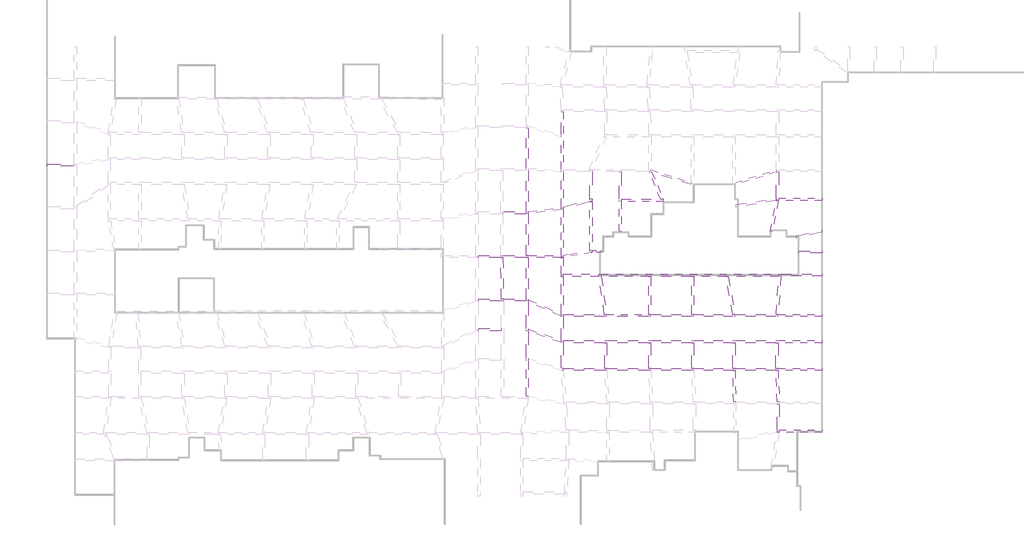
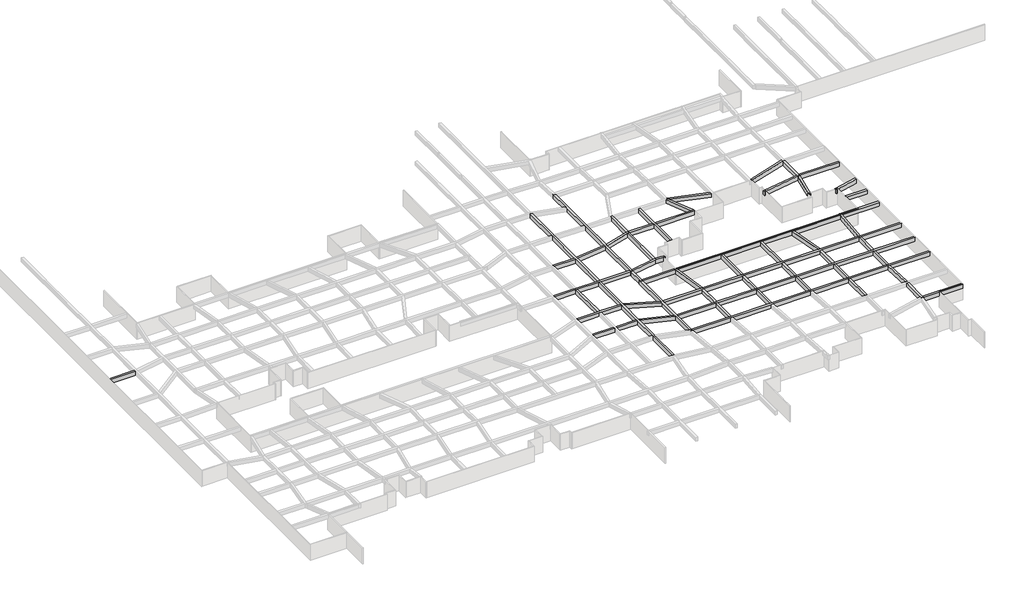
# One storey, part 13 of 45: 50 beams.
"""IFC4 building model written with IfcOpenShell, lengths in millimetres."""

import ifcopenshell
import ifcopenshell.guid

model = None  # the IFC model being written
_history = None  # IfcOwnerHistory: only IFC2X3 demands one
_inside = {}  # id of a spatial element -> (the spatial element, [elements in it])
_under = {}  # id of a project, library or spatial element -> (it, [spatial elements below it])
_declared = {}  # id of a project -> (the project, [libraries it declares])
_typed = {}  # id of a type object -> (the type object, [elements of that type])
_made_of = {}  # id of a material, layer set ... -> (it, [elements and type objects made of it])


def new_model(schema):
    """Start an empty IFC model of exactly this schema.

    Asked for "IFC4X3", IfcOpenShell would pick the latest addendum, in which some entities
    have other attributes; the version numbers below select the first issue.
    IFC2X3 requires an IfcOwnerHistory on every rooted entity: one is made here for all.
    """
    global model, _history
    if schema == "IFC4X3":
        model = ifcopenshell.file(schema_version=(4, 3, 0, 0))
    else:
        model = ifcopenshell.file(schema=schema)
    _inside.clear()
    _under.clear()
    _declared.clear()
    _typed.clear()
    _made_of.clear()
    _history = None
    if model.schema == "IFC2X3":
        org = make("IfcOrganization", Name="unknown")
        user = make(
            "IfcPersonAndOrganization",
            ThePerson=make("IfcPerson", FamilyName="unknown"),
            TheOrganization=org,
        )
        app = make(
            "IfcApplication",
            ApplicationDeveloper=org,
            Version="unknown",
            ApplicationFullName="unknown",
            ApplicationIdentifier="unknown",
        )
        _history = make(
            "IfcOwnerHistory",
            OwningUser=user,
            OwningApplication=app,
            ChangeAction="ADDED",
            CreationDate=0,
        )
    return model


def make(cls, **values):
    """One entity of the class cls with the attributes given. An attribute that is None is left unset."""
    return model.create_entity(
        cls, **{name: value for name, value in values.items() if value is not None}
    )


def rooted(cls, **values):
    """An entity with a GlobalId (a new one), such as an element, a storey or a relation."""
    return make(cls, GlobalId=ifcopenshell.guid.new(), OwnerHistory=_history, **values)


def si_unit(unit_type, name, prefix=None):
    """IfcSIUnit, for example si_unit("LENGTHUNIT", "METRE", prefix="MILLI")."""
    return make("IfcSIUnit", UnitType=unit_type, Prefix=prefix, Name=name)


def assignment(units):
    """IfcUnitAssignment: the units of a project."""
    return None if units is None else make("IfcUnitAssignment", Units=units)


def point(xyz):
    """IfcCartesianPoint."""
    return None if xyz is None else make("IfcCartesianPoint", Coordinates=xyz)


def direction(xyz):
    """IfcDirection."""
    return None if xyz is None else make("IfcDirection", DirectionRatios=xyz)


def frame(location, z_axis=None, x_axis=None):
    """IfcAxis2Placement3D, a coordinate frame: its origin and axes. An axis left out is left unset."""
    return make(
        "IfcAxis2Placement3D",
        Location=point(location),
        Axis=direction(z_axis),
        RefDirection=direction(x_axis),
    )


def origin():
    """The frame at (0, 0, 0) with its axes left unset."""
    return frame((0.0, 0.0, 0.0))


def place(relative_to, where):
    """IfcLocalPlacement: puts the frame where relative to a parent placement (None: the world)."""
    return make(
        "IfcLocalPlacement", PlacementRelTo=relative_to, RelativePlacement=where
    )


def context(
    kind, dimensions, precision=None, world=None, true_north=None, identifier=None
):
    """IfcGeometricRepresentationContext, for example the 3D "Model" context."""
    return make(
        "IfcGeometricRepresentationContext",
        ContextIdentifier=identifier,
        ContextType=kind,
        CoordinateSpaceDimension=dimensions,
        Precision=precision,
        WorldCoordinateSystem=world,
        TrueNorth=true_north,
    )


def project(units=None, contexts=None):
    """IfcProject with its units and contexts."""
    return rooted(
        "IfcProject",
        Name="project",
        RepresentationContexts=contexts,
        UnitsInContext=assignment(units),
    )


def spatial(cls, under=None, at=None, **own):
    """A site, building, storey or space (cls), placed at a placement, below another one or the project."""
    s = rooted(cls, ObjectPlacement=at, **own)
    if under is not None:
        _under.setdefault(under.id(), (under, []))[1].append(s)
    return s


def polyline(points):
    """IfcPolyline through the points."""
    return make("IfcPolyline", Points=[point(p) for p in points])


def outline(outer, holes=None, kind="AREA"):
    """IfcArbitraryClosedProfileDef: a profile drawn as a closed curve; with holes, ...WithVoids."""
    if holes is None:
        return make("IfcArbitraryClosedProfileDef", ProfileType=kind, OuterCurve=outer)
    return make(
        "IfcArbitraryProfileDefWithVoids",
        ProfileType=kind,
        OuterCurve=outer,
        InnerCurves=holes,
    )


def extrude(swept, where, along, depth):
    """IfcExtrudedAreaSolid: the profile swept, set in the frame where, extruded along a direction by depth."""
    return make(
        "IfcExtrudedAreaSolid",
        SweptArea=swept,
        Position=where,
        ExtrudedDirection=direction(along),
        Depth=depth,
    )


def faces_of(points, faces, orient=None, outer=None):
    """IfcFace entities. A face is a list of loops; a loop is a list of indices into points, from 0.

    orient and outer hold one flag for each loop. By default every Orientation is true, the
    first loop of a face is its IfcFaceOuterBound and the others are IfcFaceBound.
    """
    made = []
    for i, loops in enumerate(faces):
        bounds = []
        for j, loop in enumerate(loops):
            is_outer = j == 0 if outer is None else outer[i][j]
            bounds.append(
                make(
                    "IfcFaceOuterBound" if is_outer else "IfcFaceBound",
                    Bound=make("IfcPolyLoop", Polygon=[points[k] for k in loop]),
                    Orientation=True if orient is None else orient[i][j],
                )
            )
        made.append(make("IfcFace", Bounds=bounds))
    return made


def faceted_brep(points, faces, orient=None, outer=None, voids=None):
    """IfcFacetedBrep: a solid bounded by flat faces; with voids (closed shells), ...WithVoids."""
    shared = [point(p) for p in points]
    hull = make("IfcClosedShell", CfsFaces=faces_of(shared, faces, orient, outer))
    if voids is None:
        return make("IfcFacetedBrep", Outer=hull)
    return make(
        "IfcFacetedBrepWithVoids",
        Outer=hull,
        Voids=[
            make(cls, CfsFaces=faces_of(shared, fs, o, b)) for cls, fs, o, b in voids
        ],
    )


def shape(context_of_items, identifier, shape_type, items):
    """IfcShapeRepresentation: the items that make up one representation, for example the "Body"."""
    return make(
        "IfcShapeRepresentation",
        ContextOfItems=context_of_items,
        RepresentationIdentifier=identifier,
        RepresentationType=shape_type,
        Items=items,
    )


def source(mapping_origin, context_of_items, identifier, shape_type, items):
    """IfcRepresentationMap: a shape defined once, which mapped items show again and again."""
    return make(
        "IfcRepresentationMap",
        MappingOrigin=mapping_origin,
        MappedRepresentation=shape(context_of_items, identifier, shape_type, items),
    )


def transform(
    local_origin,
    x_axis=None,
    y_axis=None,
    z_axis=None,
    scale=None,
    scale2=None,
    scale3=None,
    uniform=True,
):
    """IfcCartesianTransformationOperator3D, or its non-uniform kind. x_axis, y_axis, z_axis: its Axis1, 2, 3."""
    if uniform:
        return make(
            "IfcCartesianTransformationOperator3D",
            Axis1=direction(x_axis),
            Axis2=direction(y_axis),
            LocalOrigin=point(local_origin),
            Scale=scale,
            Axis3=direction(z_axis),
        )
    return make(
        "IfcCartesianTransformationOperator3DnonUniform",
        Axis1=direction(x_axis),
        Axis2=direction(y_axis),
        LocalOrigin=point(local_origin),
        Scale=scale,
        Axis3=direction(z_axis),
        Scale2=scale2,
        Scale3=scale3,
    )


def mapped(mapping_source, mapping_target):
    """IfcMappedItem: shows the shape of a source again, moved by a transform."""
    return make(
        "IfcMappedItem", MappingSource=mapping_source, MappingTarget=mapping_target
    )


def made_of(thing, what):
    """Note that an element or type object is made of a material, layer set ...; save() writes the relation."""
    if what is not None:
        _made_of.setdefault(what.id(), (what, []))[1].append(thing)
    return thing


def element(
    cls,
    number,
    at=None,
    inside=None,
    cuts=None,
    type_object=None,
    material=None,
    context=None,
    identifier="Body",
    shape_type=None,
    held_by="IfcProductDefinitionShape",
    body=None,
    shapes=None,
    **own,
):
    """One element of the class cls, such as IfcWall. Its Tag is "e" and its number.

    at: its placement. inside: the storey or other place that contains it. cuts: it is an
    opening in that element (IfcRelVoidsElement). A single representation is given by context,
    identifier, shape_type and body (its items); several are given by shapes. held_by: the class
    of the entity that holds the representations. save() writes the other relations.
    """
    e = rooted(cls, Tag="e%d" % number, ObjectPlacement=at, **own)
    if body is not None:
        shapes = [shape(context, identifier, shape_type, body)]
    if shapes is not None:
        e.Representation = make(held_by, Representations=shapes)
    if inside is not None:
        _inside.setdefault(inside.id(), (inside, []))[1].append(e)
    if cuts is not None:
        rooted(
            "IfcRelVoidsElement", RelatingBuildingElement=cuts, RelatedOpeningElement=e
        )
    if type_object is not None:
        _typed.setdefault(type_object.id(), (type_object, []))[1].append(e)
    return made_of(e, material)


def aggregate(whole, parts):
    """IfcRelAggregates: a whole, such as a stair, and the parts it consists of."""
    return rooted("IfcRelAggregates", RelatingObject=whole, RelatedObjects=parts)


def save(model, path):
    """Write the relations noted so far, then the file.

    IfcRelAggregates (storeys below a building ...), IfcRelContainedInSpatialStructure (elements
    in a storey), IfcRelDefinesByType, IfcRelAssociatesMaterial and IfcRelDeclares: one each for
    every whole, place, type object, material and project.
    """
    for whole, parts in _under.values():
        aggregate(whole, parts)
    for where, things in _inside.values():
        rooted(
            "IfcRelContainedInSpatialStructure",
            RelatedElements=things,
            RelatingStructure=where,
        )
    for kind, things in _typed.values():
        rooted("IfcRelDefinesByType", RelatedObjects=things, RelatingType=kind)
    for what, things in _made_of.values():
        rooted("IfcRelAssociatesMaterial", RelatedObjects=things, RelatingMaterial=what)
    for by, libraries in _declared.values():
        rooted("IfcRelDeclares", RelatingContext=by, RelatedDefinitions=libraries)
    model.write(path)


def kl_beam_52378874(model_context):
    return source(origin(), model_context, "Body", "SweptSolid", [
        extrude(outline(polyline([(2121.5, 200.0), (2121.5, -200.0), (-2121.5, -200.0), (-2121.5, 200.0), (2121.5, 200.0)])), frame((0.0, 0.0, -400.0), z_axis=(0.0, 0.0, 1.0), x_axis=(1.0, 0.0, 0.0)), (0.0, 0.0, 1.0), 800.0),
    ])


def kl_beam_6fd21aec(model_context):
    return source(origin(), model_context, "Body", "SweptSolid", [
        extrude(outline(polyline([(2394.5, 200.0), (2394.5, -200.0), (-2394.5, -200.0), (-2394.5, 200.0), (2394.5, 200.0)])), frame((0.0, 0.0, -400.0), z_axis=(0.0, 0.0, 1.0), x_axis=(1.0, 0.0, 0.0)), (0.0, 0.0, 1.0), 800.0),
    ])


model = new_model("IFC4")

# Units and contexts
model_context = context("Model", 3, world=origin())
ifc_project = project(units=[si_unit("LENGTHUNIT", "METRE", prefix="MILLI")], contexts=[model_context])

# Site, building, storey
site = spatial("IfcSite", under=ifc_project)
building = spatial("IfcBuilding", under=site)
storey = spatial("IfcBuildingStorey", under=building, Name="户型图", Elevation=0.0)

# Beams
placement = place(None, origin())
element("IfcBeam", 1, ObjectType="KL_beam", at=placement, inside=storey, context=model_context, shape_type="SweptSolid", body=[
    extrude(outline(polyline([(-145640.2964556, -126946.3745528), (-145640.2964556, -126546.3745528), (-140635.0712547, -126546.3745528), (-140635.0712547, -126946.3745528), (-145640.2964556, -126946.3745528)])), frame((0.0, 0.0, 2500.0), z_axis=(0.0, 0.0, 1.0), x_axis=(1.0, 0.0, 0.0)), (0.0, 0.0, 1.0), 800.0),
])
element("IfcBeam", 2, ObjectType="KL_beam", at=placement, inside=storey, context=model_context, shape_type="SweptSolid", body=[
    extrude(outline(polyline([(-62877.6696197, -135611.286122), (-62877.6696197, -135211.286122), (-58630.7823984, -135211.286122), (-58630.7823984, -135611.286122), (-62877.6696197, -135611.286122)])), frame((0.0, 0.0, 2500.0), z_axis=(0.0, 0.0, 1.0), x_axis=(1.0, 0.0, 0.0)), (0.0, 0.0, 1.0), 800.0),
])
element("IfcBeam", 3, ObjectType="KL_beam", at=placement, inside=storey, context=model_context, shape_type="SweptSolid", body=[
    extrude(outline(polyline([(-58230.7823984, -135588.2311749), (-58230.7823984, -135185.2272447), (-52297.3620817, -134456.6948365), (-52297.3620817, -134859.6987667), (-58230.7823984, -135588.2311749)])), frame((0.0, 0.0, 2500.0), z_axis=(0.0, 0.0, 1.0), x_axis=(1.0, 0.0, 0.0)), (0.0, 0.0, 1.0), 800.0),
])
element("IfcBeam", 4, ObjectType="KL_beam", at=placement, inside=storey, context=model_context, shape_type="Brep", body=[
    faceted_brep([(-46687.6738698, -132877.4716384, 3300.0), (-46687.6738698, -132877.4716384, 2500.0), (-47087.6738698, -132992.1697928, 2500.0), (-51897.3620817, -134371.3256945, 2500.0), (-51897.3620817, -134371.3256945, 3300.0), (-47087.6738698, -132992.1697928, 3300.0), (-46687.6738698, -132942.8806028, 3300.0), (-46687.6738698, -133293.5914128, 3300.0), (-46687.6738698, -133293.5914128, 2500.0), (-46687.6738698, -132942.8806028, 2500.0), (-51897.3620817, -134787.4454688, 2500.0), (-51897.3620817, -134787.4454688, 3300.0), (-47087.4987798, -133408.2393608, 3300.0), (-46859.5657029, -133342.8806028, 3300.0), (-47087.4987798, -133408.2393608, 2500.0), (-46859.5657029, -133342.8806028, 2500.0)], [[[0, 1, 2, 3, 4, 5]], [[0, 6, 7, 8, 9, 1]], [[4, 3, 10, 11]], [[7, 6, 0, 5, 4, 11, 12, 13]], [[8, 7, 13, 12, 11, 10, 14, 15]], [[1, 9, 8, 15, 14, 10, 3, 2]]]),
])
element("IfcBeam", 5, ObjectType="KL_beam", at=placement, inside=storey, context=model_context, shape_type="Brep", body=[
    faceted_brep([(-46687.6738698, -127542.8806028, 3300.0), (-46784.6415945, -127542.8806028, 3300.0), (-47087.6738698, -127542.8806028, 3300.0), (-47087.6738698, -127942.8806028, 3300.0), (-47087.6738698, -132992.1697928, 3300.0), (-46687.6738698, -132877.4716384, 3300.0), (-46687.6738698, -127942.8806028, 3300.0), (-46687.6738698, -127542.8806028, 2500.0), (-46687.6738698, -132877.4716384, 2500.0), (-46687.6738698, -127942.8806028, 2500.0), (-47087.6738698, -127542.8806028, 2500.0), (-46784.6415945, -127542.8806028, 2500.0), (-47087.6738698, -132992.1697928, 2500.0), (-47087.6738698, -127942.8806028, 2500.0)], [[[0, 1, 2, 3, 4, 5, 6]], [[7, 0, 6, 5, 8, 9]], [[10, 11, 7, 9, 8, 12, 13]], [[2, 10, 13, 12, 4, 3]], [[5, 4, 12, 8]], [[2, 1, 0, 7, 11, 10]]]),
])
element("IfcBeam", 6, ObjectType="KL_beam", at=placement, inside=storey, context=model_context, shape_type="Brep", body=[
    faceted_brep([(-58457.1128979, -119970.4077047, 3300.0), (-58630.7823984, -119970.4077047, 3300.0), (-58630.7823984, -127365.3480623, 3300.0), (-58630.7823984, -127765.3480623, 3300.0), (-58630.7823984, -135211.286122, 3300.0), (-58630.7823984, -135611.286122, 3300.0), (-58630.7823984, -143149.8954633, 3300.0), (-58230.7823984, -143149.8954633, 3300.0), (-58230.7823984, -135588.2311749, 3300.0), (-58230.7823984, -135185.2272447, 3300.0), (-58230.7823984, -127768.9840855, 3300.0), (-58230.7823984, -127368.7402678, 3300.0), (-58230.7823984, -120031.0527792, 3300.0), (-58630.7823984, -119970.4077047, 2500.0), (-58630.7823984, -127365.3480623, 2500.0), (-58630.7823984, -127765.3480623, 2500.0), (-58630.7823984, -135211.286122, 2500.0), (-58630.7823984, -135611.286122, 2500.0), (-58630.7823984, -143149.8954633, 2500.0), (-58457.1128979, -119970.4077047, 2500.0), (-58230.7823984, -120031.0527792, 2500.0), (-58230.7823984, -127368.7402678, 2500.0), (-58230.7823984, -127768.9840855, 2500.0), (-58230.7823984, -135185.2272447, 2500.0), (-58230.7823984, -135588.2311749, 2500.0), (-58230.7823984, -143149.8954633, 2500.0)], [[[0, 1, 2, 3, 4, 5, 6, 7, 8, 9, 10, 11, 12]], [[1, 13, 14, 15, 16, 17, 18, 6, 5, 4, 3, 2]], [[13, 19, 20, 21, 22, 23, 24, 25, 18, 17, 16, 15, 14]], [[20, 12, 11, 10, 9, 8, 7, 25, 24, 23, 22, 21]], [[1, 0, 19, 13]], [[0, 12, 20, 19]], [[7, 6, 18, 25]]]),
])
element("IfcBeam", 7, ObjectType="KL_beam", at=placement, inside=storey, context=model_context, shape_type="Brep", body=[
    faceted_brep([(-52287.0303654, -117068.4603553, 3300.0), (-52297.3620817, -116871.3194631, 3300.0), (-52297.3620817, -121206.7974893, 3300.0), (-52297.3620817, -121620.9079614, 3300.0), (-52297.3620817, -127575.9398709, 3300.0), (-52297.3620817, -127976.1836887, 3300.0), (-52297.3620817, -134456.6948365, 3300.0), (-52297.3620817, -134859.6987667, 3300.0), (-52297.3620817, -143149.8954633, 3300.0), (-52297.3620817, -143549.8954633, 3300.0), (-52079.864349, -143549.8954633, 3300.0), (-51897.3620817, -143549.8954633, 3300.0), (-51897.3620817, -143517.7153895, 3300.0), (-51897.3620817, -143111.5447447, 3300.0), (-51897.3620817, -134787.4454688, 3300.0), (-51897.3620817, -134371.3256945, 3300.0), (-51897.3620817, -127942.8806028, 3300.0), (-51897.3620817, -127542.8806028, 3300.0), (-51897.3620817, -117068.4603553, 3300.0), (-52297.3620817, -116871.3194631, 2500.0), (-52297.3620817, -121206.7974893, 2500.0), (-52297.3620817, -121620.9079614, 2500.0), (-52297.3620817, -127575.9398709, 2500.0), (-52297.3620817, -127976.1836887, 2500.0), (-52297.3620817, -134456.6948365, 2500.0), (-52297.3620817, -134859.6987667, 2500.0), (-52297.3620817, -143149.8954633, 2500.0), (-52297.3620817, -143549.8954633, 2500.0), (-52287.0303654, -117068.4603553, 2500.0), (-51897.3620817, -117068.4603553, 2500.0), (-51897.3620817, -127542.8806028, 2500.0), (-51897.3620817, -127942.8806028, 2500.0), (-51897.3620817, -134371.3256945, 2500.0), (-51897.3620817, -134787.4454688, 2500.0), (-51897.3620817, -143111.5447447, 2500.0), (-51897.3620817, -143517.7153895, 2500.0), (-51897.3620817, -143549.8954633, 2500.0), (-52079.864349, -143549.8954633, 2500.0)], [[[0, 1, 2, 3, 4, 5, 6, 7, 8, 9, 10, 11, 12, 13, 14, 15, 16, 17, 18]], [[1, 19, 20, 21, 22, 23, 24, 25, 26, 27, 9, 8, 7, 6, 5, 4, 3, 2]], [[19, 28, 29, 30, 31, 32, 33, 34, 35, 36, 37, 27, 26, 25, 24, 23, 22, 21, 20]], [[29, 18, 17, 16, 15, 14, 13, 12, 11, 36, 35, 34, 33, 32, 31, 30]], [[0, 28, 19, 1]], [[28, 0, 18, 29]], [[11, 10, 9, 27, 37, 36]]]),
])
element("IfcBeam", 8, ObjectType="KL_beam", at=placement, inside=storey, context=model_context, shape_type="Brep", body=[
    faceted_brep([(-41387.6738698, -138842.8806028, 3300.0), (-41787.6738698, -138842.8806028, 3300.0), (-41787.6738698, -138842.8806028, 2500.0), (-41387.6738698, -138842.8806028, 2500.0), (-41387.6738698, -133342.8806028, 3300.0), (-41387.6738698, -132942.8806028, 3300.0), (-41387.6738698, -127942.8806028, 3300.0), (-41787.6738698, -127942.8806028, 3300.0), (-41787.6738698, -132942.8806028, 3300.0), (-41787.6738698, -133342.8806028, 3300.0), (-41787.6738698, -127942.8806028, 2500.0), (-41787.6738698, -132942.8806028, 2500.0), (-41787.6738698, -133342.8806028, 2500.0), (-41387.6738698, -127942.8806028, 2500.0), (-41387.6738698, -132942.8806028, 2500.0), (-41387.6738698, -133342.8806028, 2500.0)], [[[0, 1, 2, 3]], [[1, 0, 4, 5, 6, 7, 8, 9]], [[2, 1, 9, 8, 7, 10, 11, 12]], [[3, 2, 12, 11, 10, 13, 14, 15]], [[0, 3, 15, 14, 13, 6, 5, 4]], [[7, 6, 13, 10]]]),
])
element("IfcBeam", 9, ObjectType="KL_beam", at=placement, inside=storey, context=model_context, shape_type="Brep", body=[
    faceted_brep([(-33763.13275, -133342.8806028, 3300.0), (-33763.13275, -132942.8806028, 3300.0), (-34197.676901, -132942.8806028, 3300.0), (-41387.6738698, -132942.8806028, 3300.0), (-41387.6738698, -133342.8806028, 3300.0), (-33763.13275, -133342.8806028, 2500.0), (-41387.6738698, -133342.8806028, 2500.0), (-33763.13275, -132942.8806028, 2500.0), (-41387.6738698, -132942.8806028, 2500.0), (-34197.676901, -132942.8806028, 2500.0)], [[[0, 1, 2, 3, 4]], [[5, 0, 4, 6]], [[7, 5, 6, 8, 9]], [[1, 7, 9, 8, 3, 2]], [[4, 3, 8, 6]], [[1, 0, 5, 7]]]),
    faceted_brep([(-46687.6738698, -133293.5914128, 3300.0), (-46687.6738698, -133293.5914128, 2500.0), (-46859.5657029, -133342.8806028, 2500.0), (-46859.5657029, -133342.8806028, 3300.0), (-46687.6738698, -132942.8806028, 3300.0), (-46687.6738698, -132942.8806028, 2500.0), (-41787.6738698, -132942.8806028, 3300.0), (-41787.6738698, -133342.8806028, 3300.0), (-41787.6738698, -133342.8806028, 2500.0), (-41787.6738698, -132942.8806028, 2500.0), (-46687.4987798, -133342.8806028, 3300.0), (-46687.4987798, -133342.8806028, 2500.0)], [[[0, 1, 2, 3]], [[1, 0, 4, 5]], [[6, 7, 8, 9]], [[0, 3, 10, 7, 6, 4]], [[3, 2, 11, 8, 7, 10]], [[2, 1, 5, 9, 8, 11]], [[5, 4, 6, 9]]]),
])
element("IfcBeam", 10, ObjectType="KL_beam", at=placement, inside=storey, context=model_context, shape_type="Brep", body=[
    faceted_brep([(-33763.13275, -132942.8806028, 3300.0), (-35834.2157168, -128063.7148958, 3300.0), (-35987.6738698, -127702.1901429, 3300.0), (-35987.6738698, -127942.8806028, 3300.0), (-36320.0509821, -127942.8806028, 3300.0), (-34197.676901, -132942.8806028, 3300.0), (-36320.0509821, -127942.8806028, 2500.0), (-34197.676901, -132942.8806028, 2500.0), (-35987.6738698, -127702.1901429, 2500.0), (-35834.2157168, -128063.7148958, 2500.0), (-33763.13275, -132942.8806028, 2500.0), (-35987.6738698, -127942.8806028, 2500.0)], [[[0, 1, 2, 3, 4, 5]], [[4, 6, 7, 5]], [[8, 9, 10, 7, 6, 11]], [[2, 1, 0, 10, 9, 8]], [[3, 11, 6, 4]], [[11, 3, 2, 8]], [[0, 5, 7, 10]]]),
])
element("IfcBeam", 11, ObjectType="KL_beam", at=placement, inside=storey, context=model_context, shape_type="SweptSolid", body=[
    extrude(outline(polyline([(-28676.0008118, -130315.2135015), (-35834.2157168, -128063.7148958), (-35987.6738698, -127702.1901429), (-35987.6738698, -127596.1274566), (-28676.0008118, -129895.8937969), (-28676.0008118, -130315.2135015)])), frame((0.0, 0.0, 2500.0), z_axis=(0.0, 0.0, 1.0), x_axis=(1.0, 0.0, 0.0)), (0.0, 0.0, 1.0), 800.0),
])
element("IfcBeam", 12, ObjectType="KL_beam", at=placement, inside=storey, context=model_context, shape_type="SweptSolid", body=[
    extrude(outline(polyline([(-20732.9657871, -130306.3734968), (-20732.9657871, -129888.3518932), (-13240.9657871, -127614.2135527), (-13240.9657871, -128032.2351563), (-20732.9657871, -130306.3734968)])), frame((0.0, 0.0, 2500.0), z_axis=(0.0, 0.0, 1.0), x_axis=(1.0, 0.0, 0.0)), (0.0, 0.0, 1.0), 800.0),
])
element("IfcBeam", 13, ObjectType="KL_beam", at=placement, inside=storey, context=model_context, shape_type="Brep", body=[
    faceted_brep([(-13240.9657871, -133162.5159097, 3300.0), (-13025.0033804, -133162.5159097, 3300.0), (-12875.8764446, -133162.5159097, 3300.0), (-12840.9657871, -133162.5159097, 3300.0), (-12840.9657871, -132762.5159097, 3300.0), (-12840.9657871, -127962.1982562, 3300.0), (-13010.2338015, -127962.1982562, 3300.0), (-13240.9657871, -128032.2351563, 3300.0), (-13240.9657871, -132791.7349443, 3300.0), (-13240.9657871, -128032.2351563, 2500.0), (-13240.9657871, -132791.7349443, 2500.0), (-13240.9657871, -133162.5159097, 2500.0), (-12840.9657871, -133162.5159097, 2500.0), (-12875.8764446, -133162.5159097, 2500.0), (-13025.0033804, -133162.5159097, 2500.0), (-13010.2338015, -127962.1982562, 2500.0), (-12840.9657871, -127962.1982562, 2500.0), (-12840.9657871, -132762.5159097, 2500.0)], [[[0, 1, 2, 3, 4, 5, 6, 7, 8]], [[7, 9, 10, 11, 0, 8]], [[12, 13, 14, 11, 10, 9, 15, 16, 17]], [[3, 12, 17, 16, 5, 4]], [[9, 7, 6, 15]], [[6, 5, 16, 15]], [[3, 2, 1, 0, 11, 14, 13, 12]]]),
])
element("IfcBeam", 14, ObjectType="KL_beam", at=placement, inside=storey, context=model_context, shape_type="SweptSolid", body=[
    extrude(outline(polyline([(-4940.7437218, -132762.5159097), (-4940.7437218, -133162.5159097), (-12840.9657871, -133162.5159097), (-12840.9657871, -132762.5159097), (-4940.7437218, -132762.5159097)])), frame((0.0, 0.0, 2500.0), z_axis=(0.0, 0.0, 1.0), x_axis=(1.0, 0.0, 0.0)), (0.0, 0.0, 1.0), 800.0),
])
element("IfcBeam", 15, ObjectType="KL_beam", at=placement, inside=storey, context=model_context, shape_type="Brep", body=[
    faceted_brep([(-20515.8882173, -134348.9555121, 3300.0), (-20578.4620033, -133953.8801759, 3300.0), (-20578.4620033, -133953.8801759, 2500.0), (-20515.8882173, -134348.9555121, 2500.0), (-13291.5698558, -133204.7358917, 3300.0), (-13025.0033804, -133162.5159097, 3300.0), (-13240.9657871, -133162.5159097, 3300.0), (-13240.9657871, -132791.7349443, 3300.0), (-13240.9657871, -132791.7349443, 2500.0), (-13240.9657871, -133162.5159097, 2500.0), (-13025.0033804, -133162.5159097, 2500.0), (-13291.5698558, -133204.7358917, 2500.0)], [[[0, 1, 2, 3]], [[1, 0, 4, 5, 6, 7]], [[2, 1, 7, 8]], [[3, 2, 8, 9, 10, 11]], [[0, 3, 11, 10, 5, 4]], [[9, 6, 5, 10]], [[6, 9, 8, 7]]]),
])
element("IfcBeam", 16, ObjectType="KL_beam", at=placement, inside=storey, context=model_context, shape_type="Brep", body=[
    faceted_brep([(-52297.3620817, -143549.8954633, 3300.0), (-52297.3620817, -143149.8954633, 3300.0), (-58230.7823984, -143149.8954633, 3300.0), (-58630.7823984, -143149.8954633, 3300.0), (-62877.6696197, -143149.8954633, 3300.0), (-63277.6696197, -143149.8954633, 3300.0), (-67364.0267672, -143149.8954633, 3300.0), (-67364.0267672, -143549.8954633, 3300.0), (-67363.6944245, -143549.8954633, 3300.0), (-63274.2046125, -143549.8954633, 3300.0), (-62874.1436813, -143549.8954633, 3300.0), (-58663.6944245, -143549.8954633, 3300.0), (-58263.6944245, -143549.8954633, 3300.0), (-52297.3620817, -143549.8954633, 2500.0), (-67364.0267672, -143549.8954633, 2500.0), (-67363.6944245, -143549.8954633, 2500.0), (-63274.2046125, -143549.8954633, 2500.0), (-62874.1436813, -143549.8954633, 2500.0), (-58663.6944245, -143549.8954633, 2500.0), (-58263.6944245, -143549.8954633, 2500.0), (-52297.3620817, -143149.8954633, 2500.0), (-67364.0267672, -143149.8954633, 2500.0), (-63277.6696197, -143149.8954633, 2500.0), (-62877.6696197, -143149.8954633, 2500.0), (-58630.7823984, -143149.8954633, 2500.0), (-58230.7823984, -143149.8954633, 2500.0)], [[[0, 1, 2, 3, 4, 5, 6, 7, 8, 9, 10, 11, 12]], [[13, 0, 12, 11, 10, 9, 8, 7, 14, 15, 16, 17, 18, 19]], [[20, 13, 19, 18, 17, 16, 15, 14, 21, 22, 23, 24, 25]], [[1, 20, 25, 24, 23, 22, 21, 6, 5, 4, 3, 2]], [[1, 0, 13, 20]], [[7, 6, 21, 14]]]),
])
element("IfcBeam", 17, ObjectType="KL_beam", at=placement, inside=storey, context=model_context, shape_type="Brep", body=[
    faceted_brep([(-52079.864349, -143549.8954633, 3300.0), (-52297.3620817, -143549.8954633, 3300.0), (-52297.3620817, -143588.2461818, 3300.0), (-52297.3620817, -143588.2461818, 2500.0), (-52079.864349, -143549.8954633, 2500.0), (-52297.3620817, -143549.8954633, 2500.0)], [[[0, 1, 2]], [[2, 3, 4, 0]], [[5, 4, 3]], [[3, 2, 1, 5]], [[1, 0, 4, 5]]]),
    faceted_brep([(-51897.3620817, -143111.5447447, 2500.0), (-51897.3620817, -143111.5447447, 3300.0), (-47087.4987798, -142263.4360711, 3300.0), (-46687.4987798, -142192.9052788, 3300.0), (-46687.4987798, -142192.9052788, 2500.0), (-47087.4987798, -142263.4360711, 2500.0), (-51897.3620817, -143517.7153895, 2500.0), (-51897.3620817, -143517.7153895, 3300.0), (-51897.3620817, -143149.8954633, 3300.0), (-51897.3620817, -143149.8954633, 2500.0), (-46687.4987798, -142599.0759236, 3300.0), (-46687.4987798, -142231.0431969, 3300.0), (-46868.794196, -142631.0431969, 3300.0), (-46868.794196, -142631.0431969, 2500.0), (-46687.4987798, -142599.0759236, 2500.0), (-46687.4987798, -142231.0431969, 2500.0)], [[[0, 1, 2, 3, 4, 5]], [[6, 7, 8, 1, 0, 9]], [[10, 11, 3, 2, 1, 8, 7, 12]], [[7, 6, 13, 14, 10, 12]], [[4, 15, 14, 13, 6, 9, 0, 5]], [[3, 11, 10, 14, 15, 4]]]),
])
element("IfcBeam", 18, ObjectType="KL_beam", at=placement, inside=storey, context=model_context, shape_type="Brep", body=[
    faceted_brep([(-52297.3620817, -146946.58821, 3300.0), (-51919.3672313, -146946.58821, 3300.0), (-51897.3620817, -146946.58821, 3300.0), (-51897.3620817, -146546.58821, 3300.0), (-51897.3620817, -143549.8954633, 3300.0), (-52079.864349, -143549.8954633, 3300.0), (-52297.3620817, -143588.2461818, 3300.0), (-52297.3620817, -146546.58821, 3300.0), (-52297.3620817, -146946.58821, 2500.0), (-52297.3620817, -143588.2461818, 2500.0), (-52297.3620817, -146546.58821, 2500.0), (-51897.3620817, -146946.58821, 2500.0), (-51919.3672313, -146946.58821, 2500.0), (-52079.864349, -143549.8954633, 2500.0), (-51897.3620817, -143549.8954633, 2500.0), (-51897.3620817, -146546.58821, 2500.0)], [[[0, 1, 2, 3, 4, 5, 6, 7]], [[8, 0, 7, 6, 9, 10]], [[11, 12, 8, 10, 9, 13, 14, 15]], [[14, 4, 3, 2, 11, 15]], [[4, 14, 13, 5]], [[6, 5, 13, 9]], [[2, 1, 0, 8, 12, 11]]]),
])
element("IfcBeam", 19, ObjectType="KL_beam", at=placement, inside=storey, context=model_context, shape_type="Brep", body=[
    faceted_brep([(-58663.6944245, -168749.8954633, 3300.0), (-58263.6944245, -168749.8954633, 3300.0), (-58263.6944245, -162315.3044276, 3300.0), (-58263.6944245, -161899.1846532, 3300.0), (-58263.6944245, -156930.2851222, 3300.0), (-58263.6944245, -156507.2368497, 3300.0), (-58263.6944245, -151557.868456, 3300.0), (-58263.6944245, -151120.0139446, 3300.0), (-58263.6944245, -143549.8954633, 3300.0), (-58663.6944245, -143549.8954633, 3300.0), (-58663.6944245, -151049.8954633, 3300.0), (-58663.6944245, -151449.8954633, 3300.0), (-58663.6944245, -156449.8954633, 3300.0), (-58663.6944245, -156849.8954633, 3300.0), (-58663.6944245, -161849.8954633, 3300.0), (-58663.6944245, -162249.8954633, 3300.0), (-58263.6944245, -168749.8954633, 2500.0), (-58263.6944245, -162315.3044276, 2500.0), (-58263.6944245, -161899.1846532, 2500.0), (-58263.6944245, -156930.2851222, 2500.0), (-58263.6944245, -156507.2368497, 2500.0), (-58263.6944245, -151557.868456, 2500.0), (-58263.6944245, -151120.0139446, 2500.0), (-58263.6944245, -143549.8954633, 2500.0), (-58663.6944245, -168749.8954633, 2500.0), (-58663.6944245, -162249.8954633, 2500.0), (-58663.6944245, -161849.8954633, 2500.0), (-58663.6944245, -156849.8954633, 2500.0), (-58663.6944245, -156449.8954633, 2500.0), (-58663.6944245, -151449.8954633, 2500.0), (-58663.6944245, -151049.8954633, 2500.0), (-58663.6944245, -143549.8954633, 2500.0)], [[[0, 1, 2, 3, 4, 5, 6, 7, 8, 9, 10, 11, 12, 13, 14, 15]], [[1, 16, 17, 18, 19, 20, 21, 22, 23, 8, 7, 6, 5, 4, 3, 2]], [[16, 24, 25, 26, 27, 28, 29, 30, 31, 23, 22, 21, 20, 19, 18, 17]], [[24, 0, 15, 14, 13, 12, 11, 10, 9, 31, 30, 29, 28, 27, 26, 25]], [[1, 0, 24, 16]], [[9, 8, 23, 31]]]),
])
element("IfcBeam", 20, ObjectType="KL_beam", at=placement, inside=storey, context=model_context, shape_type="SweptSolid", body=[
    extrude(outline(polyline([(-63274.2046125, -143549.8954633), (-62874.1436813, -143549.8954633), (-62743.2306943, -151049.8954633), (-63143.2916255, -151049.8954633), (-63274.2046125, -143549.8954633)])), frame((0.0, 0.0, 2500.0), z_axis=(0.0, 0.0, 1.0), x_axis=(1.0, 0.0, 0.0)), (0.0, 0.0, 1.0), 800.0),
])
element("IfcBeam", 21, ObjectType="KL_beam", at=placement, inside=storey, context=model_context, shape_type="Brep", body=[
    faceted_brep([(-67363.6944245, -151049.8954633, 3300.0), (-67363.6944245, -151449.8954633, 3300.0), (-63139.7956089, -151449.8954633, 3300.0), (-62739.7956089, -151449.8954633, 3300.0), (-58663.6944245, -151449.8954633, 3300.0), (-58663.6944245, -151049.8954633, 3300.0), (-62743.2306943, -151049.8954633, 3300.0), (-63143.2916255, -151049.8954633, 3300.0), (-67363.6944245, -151449.8954633, 2500.0), (-63139.7956089, -151449.8954633, 2500.0), (-62739.7956089, -151449.8954633, 2500.0), (-58663.6944245, -151449.8954633, 2500.0), (-67363.6944245, -151049.8954633, 2500.0), (-63143.2916255, -151049.8954633, 2500.0), (-62743.2306943, -151049.8954633, 2500.0), (-58663.6944245, -151049.8954633, 2500.0)], [[[0, 1, 2, 3, 4, 5, 6, 7]], [[1, 8, 9, 10, 11, 4, 3, 2]], [[8, 12, 13, 14, 15, 11, 10, 9]], [[12, 0, 7, 6, 5, 15, 14, 13]], [[1, 0, 12, 8]], [[5, 4, 11, 15]]]),
])
element("IfcBeam", 22, ObjectType="KL_beam", at=placement, inside=storey, context=model_context, shape_type="SweptSolid", body=[
    extrude(outline(polyline([(-58263.6944245, -151557.868456), (-58263.6944245, -151120.0139446), (-52319.3672313, -153766.5989259), (-52319.3672313, -154204.4534373), (-58263.6944245, -151557.868456)])), frame((0.0, 0.0, 2500.0), z_axis=(0.0, 0.0, 1.0), x_axis=(1.0, 0.0, 0.0)), (0.0, 0.0, 1.0), 800.0),
])
element("IfcBeam", 23, ObjectType="KL_beam", at=placement, inside=storey, context=model_context, shape_type="SweptSolid", body=[
    extrude(outline(polyline([(-58263.6944245, -156930.2851222), (-58263.6944245, -156507.2368497), (-52319.3672313, -158554.0328447), (-52319.3672313, -158977.0811172), (-58263.6944245, -156930.2851222)])), frame((0.0, 0.0, 2500.0), z_axis=(0.0, 0.0, 1.0), x_axis=(1.0, 0.0, 0.0)), (0.0, 0.0, 1.0), 800.0),
])
element("IfcBeam", 24, ObjectType="KL_beam", at=placement, inside=storey, context=model_context, shape_type="Brep", body=[
    faceted_brep([(-51919.3672313, -163718.3912016, 3300.0), (-52020.0590892, -164069.5454413, 3300.0), (-51919.3672313, -164069.5454413, 3300.0), (-51919.3672313, -146946.58821, 2500.0), (-51919.3672313, -146946.58821, 3300.0), (-51919.3672313, -153874.5719187, 3300.0), (-51919.3672313, -154274.5719187, 3300.0), (-51919.3672313, -158634.2773576, 3300.0), (-51919.3672313, -159034.2773576, 3300.0), (-51919.3672313, -163669.5454413, 3300.0), (-51919.3672313, -164069.5454413, 2500.0), (-51919.3672313, -163718.3912016, 2500.0), (-51919.3672313, -163669.5454413, 2500.0), (-51919.3672313, -159034.2773576, 2500.0), (-51919.3672313, -158634.2773576, 2500.0), (-51919.3672313, -154274.5719187, 2500.0), (-51919.3672313, -153874.5719187, 2500.0), (-52020.0590892, -164069.5454413, 2500.0), (-52319.3672313, -163603.6930473, 2500.0), (-52319.3672313, -163603.6930473, 3300.0), (-52319.3672313, -158977.0811172, 3300.0), (-52319.3672313, -158554.0328447, 3300.0), (-52319.3672313, -154204.4534373, 3300.0), (-52319.3672313, -153766.5989259, 3300.0), (-52319.3672313, -146546.58821, 3300.0), (-52319.3672313, -146546.58821, 2500.0), (-52319.3672313, -153766.5989259, 2500.0), (-52319.3672313, -154204.4534373, 2500.0), (-52319.3672313, -158554.0328447, 2500.0), (-52319.3672313, -158977.0811172, 2500.0), (-52297.3620817, -146946.58821, 3300.0), (-52297.3620817, -146946.58821, 2500.0), (-52297.3620817, -146546.58821, 2500.0), (-52297.3620817, -146546.58821, 3300.0)], [[[0, 1, 2]], [[3, 4, 5, 6, 7, 8, 9, 0, 2, 10, 11, 12, 13, 14, 15, 16]], [[17, 11, 10]], [[18, 19, 20, 21, 22, 23, 24, 25, 26, 27, 28, 29]], [[1, 17, 10, 2]], [[11, 0, 19, 18]], [[0, 11, 17, 1]], [[30, 31, 32, 33]], [[25, 24, 33, 32]], [[31, 30, 4, 3]], [[19, 0, 9, 8, 7, 6, 5, 4, 30, 33, 24, 23, 22, 21, 20]], [[11, 18, 29, 28, 27, 26, 25, 32, 31, 3, 16, 15, 14, 13, 12]]]),
])
element("IfcBeam", 25, ObjectType="KL_beam", at=placement, inside=storey, context=model_context, shape_type="Brep", body=[
    faceted_brep([(-4940.9444439, -153874.5719187, 3300.0), (-4940.9444439, -154274.5719187, 3300.0), (-4940.9444439, -154274.5719187, 2500.0), (-4940.9444439, -153874.5719187, 2500.0), (-12904.8594516, -153874.5719187, 3300.0), (-13305.8362108, -153874.5719187, 3300.0), (-20751.547305, -153874.5719187, 3300.0), (-21157.7179498, -153874.5719187, 3300.0), (-28219.3672313, -153874.5719187, 3300.0), (-28619.3672313, -153874.5719187, 3300.0), (-36019.3672313, -153874.5719187, 3300.0), (-36419.3672313, -153874.5719187, 3300.0), (-44045.5098837, -153874.5719187, 3300.0), (-44449.4409127, -153874.5719187, 3300.0), (-51919.3672313, -153874.5719187, 3300.0), (-51919.3672313, -154274.5719187, 3300.0), (-44419.3672313, -154274.5719187, 3300.0), (-44019.3672313, -154274.5719187, 3300.0), (-36419.3672313, -154274.5719187, 3300.0), (-36019.3672313, -154274.5719187, 3300.0), (-28619.3672313, -154274.5719187, 3300.0), (-28219.3672313, -154274.5719187, 3300.0), (-21119.3672313, -154274.5719187, 3300.0), (-20719.3672313, -154274.5719187, 3300.0), (-13319.3672313, -154274.5719187, 3300.0), (-12919.3672313, -154274.5719187, 3300.0), (-51919.3672313, -154274.5719187, 2500.0), (-44419.3672313, -154274.5719187, 2500.0), (-44019.3672313, -154274.5719187, 2500.0), (-36419.3672313, -154274.5719187, 2500.0), (-36019.3672313, -154274.5719187, 2500.0), (-28619.3672313, -154274.5719187, 2500.0), (-28219.3672313, -154274.5719187, 2500.0), (-21119.3672313, -154274.5719187, 2500.0), (-20719.3672313, -154274.5719187, 2500.0), (-13319.3672313, -154274.5719187, 2500.0), (-12919.3672313, -154274.5719187, 2500.0), (-51919.3672313, -153874.5719187, 2500.0), (-44449.4409127, -153874.5719187, 2500.0), (-44045.5098837, -153874.5719187, 2500.0), (-36419.3672313, -153874.5719187, 2500.0), (-36019.3672313, -153874.5719187, 2500.0), (-28619.3672313, -153874.5719187, 2500.0), (-28219.3672313, -153874.5719187, 2500.0), (-21157.7179498, -153874.5719187, 2500.0), (-20751.547305, -153874.5719187, 2500.0), (-13305.8362108, -153874.5719187, 2500.0), (-12904.8594516, -153874.5719187, 2500.0)], [[[0, 1, 2, 3]], [[1, 0, 4, 5, 6, 7, 8, 9, 10, 11, 12, 13, 14, 15, 16, 17, 18, 19, 20, 21, 22, 23, 24, 25]], [[2, 1, 25, 24, 23, 22, 21, 20, 19, 18, 17, 16, 15, 26, 27, 28, 29, 30, 31, 32, 33, 34, 35, 36]], [[3, 2, 36, 35, 34, 33, 32, 31, 30, 29, 28, 27, 26, 37, 38, 39, 40, 41, 42, 43, 44, 45, 46, 47]], [[0, 3, 47, 46, 45, 44, 43, 42, 41, 40, 39, 38, 37, 14, 13, 12, 11, 10, 9, 8, 7, 6, 5, 4]], [[15, 14, 37, 26]]]),
])
element("IfcBeam", 26, ObjectType="KL_beam", at=placement, inside=storey, context=model_context, shape_type="Brep", body=[
    faceted_brep([(-4940.9444439, -158634.2773576, 3300.0), (-4940.9444439, -159034.2773576, 3300.0), (-4940.9444439, -159034.2773576, 2500.0), (-4940.9444439, -158634.2773576, 2500.0), (-12919.3672313, -158634.2773576, 3300.0), (-13319.3672313, -158634.2773576, 3300.0), (-20719.3672313, -158634.2773576, 3300.0), (-21119.3672313, -158634.2773576, 3300.0), (-28219.3672313, -158634.2773576, 3300.0), (-28619.3672313, -158634.2773576, 3300.0), (-36019.3672313, -158634.2773576, 3300.0), (-36419.3672313, -158634.2773576, 3300.0), (-44019.3672313, -158634.2773576, 3300.0), (-44419.3672313, -158634.2773576, 3300.0), (-51919.3672313, -158634.2773576, 3300.0), (-51919.3672313, -159034.2773576, 3300.0), (-44419.3672313, -159034.2773576, 3300.0), (-44019.3672313, -159034.2773576, 3300.0), (-36419.3672313, -159034.2773576, 3300.0), (-36019.3672313, -159034.2773576, 3300.0), (-28619.3672313, -159034.2773576, 3300.0), (-28219.3672313, -159034.2773576, 3300.0), (-21119.3672313, -159034.2773576, 3300.0), (-20719.3672313, -159034.2773576, 3300.0), (-13319.3672313, -159034.2773576, 3300.0), (-12919.3672313, -159034.2773576, 3300.0), (-51919.3672313, -159034.2773576, 2500.0), (-44419.3672313, -159034.2773576, 2500.0), (-44019.3672313, -159034.2773576, 2500.0), (-36419.3672313, -159034.2773576, 2500.0), (-36019.3672313, -159034.2773576, 2500.0), (-28619.3672313, -159034.2773576, 2500.0), (-28219.3672313, -159034.2773576, 2500.0), (-21119.3672313, -159034.2773576, 2500.0), (-20719.3672313, -159034.2773576, 2500.0), (-13319.3672313, -159034.2773576, 2500.0), (-12919.3672313, -159034.2773576, 2500.0), (-51919.3672313, -158634.2773576, 2500.0), (-44419.3672313, -158634.2773576, 2500.0), (-44019.3672313, -158634.2773576, 2500.0), (-36419.3672313, -158634.2773576, 2500.0), (-36019.3672313, -158634.2773576, 2500.0), (-28619.3672313, -158634.2773576, 2500.0), (-28219.3672313, -158634.2773576, 2500.0), (-21119.3672313, -158634.2773576, 2500.0), (-20719.3672313, -158634.2773576, 2500.0), (-13319.3672313, -158634.2773576, 2500.0), (-12919.3672313, -158634.2773576, 2500.0)], [[[0, 1, 2, 3]], [[1, 0, 4, 5, 6, 7, 8, 9, 10, 11, 12, 13, 14, 15, 16, 17, 18, 19, 20, 21, 22, 23, 24, 25]], [[2, 1, 25, 24, 23, 22, 21, 20, 19, 18, 17, 16, 15, 26, 27, 28, 29, 30, 31, 32, 33, 34, 35, 36]], [[3, 2, 36, 35, 34, 33, 32, 31, 30, 29, 28, 27, 26, 37, 38, 39, 40, 41, 42, 43, 44, 45, 46, 47]], [[0, 3, 47, 46, 45, 44, 43, 42, 41, 40, 39, 38, 37, 14, 13, 12, 11, 10, 9, 8, 7, 6, 5, 4]], [[15, 14, 37, 26]]]),
])
element("IfcBeam", 27, ObjectType="KL_beam", at=placement, inside=storey, context=model_context, shape_type="Brep", body=[
    faceted_brep([(-4940.7330502, -163669.5454413, 3300.0), (-4940.7330502, -164069.5454413, 3300.0), (-4940.7330502, -164069.5454413, 2500.0), (-4940.7330502, -163669.5454413, 2500.0), (-12919.3672313, -163669.5454413, 3300.0), (-13319.3672313, -163669.5454413, 3300.0), (-20719.3672313, -163669.5454413, 3300.0), (-21119.3672313, -163669.5454413, 3300.0), (-28219.3672313, -163669.5454413, 3300.0), (-28619.3672313, -163669.5454413, 3300.0), (-36019.3672313, -163669.5454413, 3300.0), (-36419.3672313, -163669.5454413, 3300.0), (-44019.3672313, -163669.5454413, 3300.0), (-44419.3672313, -163669.5454413, 3300.0), (-51919.3672313, -163669.5454413, 3300.0), (-51919.3672313, -163718.3912016, 3300.0), (-51919.3672313, -164069.5454413, 3300.0), (-51900.6827437, -164069.5454413, 3300.0), (-44406.0241434, -164069.5454413, 3300.0), (-44005.0752794, -164069.5454413, 3300.0), (-36409.1346345, -164069.5454413, 3300.0), (-36008.5856961, -164069.5454413, 3300.0), (-28609.1601446, -164069.5454413, 3300.0), (-28208.6112062, -164069.5454413, 3300.0), (-21115.9066839, -164069.5454413, 3300.0), (-20715.8457527, -164069.5454413, 3300.0), (-13312.5049862, -164069.5454413, 3300.0), (-12912.2611685, -164069.5454413, 3300.0), (-51919.3672313, -164069.5454413, 2500.0), (-51900.6827437, -164069.5454413, 2500.0), (-44406.0241434, -164069.5454413, 2500.0), (-44005.0752794, -164069.5454413, 2500.0), (-36409.1346345, -164069.5454413, 2500.0), (-36008.5856961, -164069.5454413, 2500.0), (-28609.1601446, -164069.5454413, 2500.0), (-28208.6112062, -164069.5454413, 2500.0), (-21115.9066839, -164069.5454413, 2500.0), (-20715.8457527, -164069.5454413, 2500.0), (-13312.5049862, -164069.5454413, 2500.0), (-12912.2611685, -164069.5454413, 2500.0), (-51919.3672313, -163718.3912016, 2500.0), (-51919.3672313, -163669.5454413, 2500.0), (-44419.3672313, -163669.5454413, 2500.0), (-44019.3672313, -163669.5454413, 2500.0), (-36419.3672313, -163669.5454413, 2500.0), (-36019.3672313, -163669.5454413, 2500.0), (-28619.3672313, -163669.5454413, 2500.0), (-28219.3672313, -163669.5454413, 2500.0), (-21119.3672313, -163669.5454413, 2500.0), (-20719.3672313, -163669.5454413, 2500.0), (-13319.3672313, -163669.5454413, 2500.0), (-12919.3672313, -163669.5454413, 2500.0)], [[[0, 1, 2, 3]], [[1, 0, 4, 5, 6, 7, 8, 9, 10, 11, 12, 13, 14, 15, 16, 17, 18, 19, 20, 21, 22, 23, 24, 25, 26, 27]], [[2, 1, 27, 26, 25, 24, 23, 22, 21, 20, 19, 18, 17, 16, 28, 29, 30, 31, 32, 33, 34, 35, 36, 37, 38, 39]], [[3, 2, 39, 38, 37, 36, 35, 34, 33, 32, 31, 30, 29, 28, 40, 41, 42, 43, 44, 45, 46, 47, 48, 49, 50, 51]], [[0, 3, 51, 50, 49, 48, 47, 46, 45, 44, 43, 42, 41, 14, 13, 12, 11, 10, 9, 8, 7, 6, 5, 4]], [[15, 14, 41, 40, 28, 16]]]),
    faceted_brep([(-52306.232201, -164023.579231, 3300.0), (-52145.9289751, -164069.5454413, 3300.0), (-52145.9289751, -164069.5454413, 2500.0), (-52306.232201, -164023.579231, 2500.0), (-52302.2106787, -164069.5454413, 3300.0), (-52302.2106787, -164069.5454413, 2500.0)], [[[0, 1, 2, 3]], [[1, 0, 4]], [[2, 1, 4, 5]], [[3, 2, 5]], [[5, 4, 0, 3]]]),
])
element("IfcBeam", 28, ObjectType="KL_beam", at=placement, inside=storey, context=model_context, shape_type="SweptSolid", body=[
    extrude(outline(polyline([(-44419.3672313, -154274.5719187), (-44019.3672313, -154274.5719187), (-44019.3672313, -158634.2773576), (-44419.3672313, -158634.2773576), (-44419.3672313, -154274.5719187)])), frame((0.0, 0.0, 2500.0), z_axis=(0.0, 0.0, 1.0), x_axis=(1.0, 0.0, 0.0)), (0.0, 0.0, 1.0), 800.0),
    extrude(outline(polyline([(-44019.3672313, -163669.5454413), (-44419.3672313, -163669.5454413), (-44419.3672313, -159034.2773576), (-44019.3672313, -159034.2773576), (-44019.3672313, -163669.5454413)])), frame((0.0, 0.0, 2500.0), z_axis=(0.0, 0.0, 1.0), x_axis=(1.0, 0.0, 0.0)), (0.0, 0.0, 1.0), 800.0),
])
element("IfcBeam", 29, ObjectType="KL_beam", at=placement, inside=storey, context=model_context, shape_type="SweptSolid", body=[
    extrude(outline(polyline([(-36419.3672313, -154274.5719187), (-36019.3672313, -154274.5719187), (-36019.3672313, -158634.2773576), (-36419.3672313, -158634.2773576), (-36419.3672313, -154274.5719187)])), frame((0.0, 0.0, 2500.0), z_axis=(0.0, 0.0, 1.0), x_axis=(1.0, 0.0, 0.0)), (0.0, 0.0, 1.0), 800.0),
    extrude(outline(polyline([(-36019.3672313, -163669.5454413), (-36419.3672313, -163669.5454413), (-36419.3672313, -159034.2773576), (-36019.3672313, -159034.2773576), (-36019.3672313, -163669.5454413)])), frame((0.0, 0.0, 2500.0), z_axis=(0.0, 0.0, 1.0), x_axis=(1.0, 0.0, 0.0)), (0.0, 0.0, 1.0), 800.0),
])
element("IfcBeam", 30, ObjectType="KL_beam", at=placement, inside=storey, context=model_context, shape_type="SweptSolid", body=[
    extrude(outline(polyline([(-28619.3672313, -154274.5719187), (-28219.3672313, -154274.5719187), (-28219.3672313, -158634.2773576), (-28619.3672313, -158634.2773576), (-28619.3672313, -154274.5719187)])), frame((0.0, 0.0, 2500.0), z_axis=(0.0, 0.0, 1.0), x_axis=(1.0, 0.0, 0.0)), (0.0, 0.0, 1.0), 800.0),
    extrude(outline(polyline([(-28219.3672313, -163669.5454413), (-28619.3672313, -163669.5454413), (-28619.3672313, -159034.2773576), (-28219.3672313, -159034.2773576), (-28219.3672313, -163669.5454413)])), frame((0.0, 0.0, 2500.0), z_axis=(0.0, 0.0, 1.0), x_axis=(1.0, 0.0, 0.0)), (0.0, 0.0, 1.0), 800.0),
])
element("IfcBeam", 31, ObjectType="KL_beam", at=placement, inside=storey, context=model_context, shape_type="SweptSolid", body=[
    extrude(outline(polyline([(-21119.3672313, -154274.5719187), (-20719.3672313, -154274.5719187), (-20719.3672313, -158634.2773576), (-21119.3672313, -158634.2773576), (-21119.3672313, -154274.5719187)])), frame((0.0, 0.0, 2500.0), z_axis=(0.0, 0.0, 1.0), x_axis=(1.0, 0.0, 0.0)), (0.0, 0.0, 1.0), 800.0),
    extrude(outline(polyline([(-20719.3672313, -163669.5454413), (-21119.3672313, -163669.5454413), (-21119.3672313, -159034.2773576), (-20719.3672313, -159034.2773576), (-20719.3672313, -163669.5454413)])), frame((0.0, 0.0, 2500.0), z_axis=(0.0, 0.0, 1.0), x_axis=(1.0, 0.0, 0.0)), (0.0, 0.0, 1.0), 800.0),
])
element("IfcBeam", 32, ObjectType="KL_beam", at=placement, inside=storey, context=model_context, shape_type="SweptSolid", body=[
    extrude(outline(polyline([(-13319.3672313, -154274.5719187), (-12919.3672313, -154274.5719187), (-12919.3672313, -158634.2773576), (-13319.3672313, -158634.2773576), (-13319.3672313, -154274.5719187)])), frame((0.0, 0.0, 2500.0), z_axis=(0.0, 0.0, 1.0), x_axis=(1.0, 0.0, 0.0)), (0.0, 0.0, 1.0), 800.0),
    extrude(outline(polyline([(-12919.3672313, -163669.5454413), (-13319.3672313, -163669.5454413), (-13319.3672313, -159034.2773576), (-12919.3672313, -159034.2773576), (-12919.3672313, -163669.5454413)])), frame((0.0, 0.0, 2500.0), z_axis=(0.0, 0.0, 1.0), x_axis=(1.0, 0.0, 0.0)), (0.0, 0.0, 1.0), 800.0),
])
element("IfcBeam", 33, ObjectType="KL_beam", at=placement, inside=storey, context=model_context, shape_type="SweptSolid", body=[
    extrude(outline(polyline([(-21115.9066839, -164069.5454413), (-20715.8457527, -164069.5454413), (-20616.7570555, -169746.3330997), (-21016.8179867, -169746.3330997), (-21115.9066839, -164069.5454413)])), frame((0.0, 0.0, 2500.0), z_axis=(0.0, 0.0, 1.0), x_axis=(1.0, 0.0, 0.0)), (0.0, 0.0, 1.0), 800.0),
])
element("IfcBeam", 34, ObjectType="KL_beam", at=placement, inside=storey, context=model_context, shape_type="SweptSolid", body=[
    extrude(outline(polyline([(-13312.5049862, -164069.5454413), (-12912.2611685, -164069.5454413), (-12714.0233753, -169746.3330997), (-13114.267193, -169746.3330997), (-13312.5049862, -164069.5454413)])), frame((0.0, 0.0, 2500.0), z_axis=(0.0, 0.0, 1.0), x_axis=(1.0, 0.0, 0.0)), (0.0, 0.0, 1.0), 800.0),
])
element("IfcBeam", 35, ObjectType="KL_beam", at=placement, inside=storey, context=model_context, shape_type="Brep", body=[
    faceted_brep([(-13107.1611302, -175246.3330997, 3300.0), (-12883.7429674, -175246.3330997, 3300.0), (-12736.0252562, -175246.3330997, 3300.0), (-12707.1611302, -175246.3330997, 3300.0), (-12707.1611302, -174846.3330997, 3300.0), (-12707.1611302, -170146.3330997, 3300.0), (-13107.1611302, -170146.3330997, 3300.0), (-13107.1611302, -174887.8218274, 3300.0), (-13107.1611302, -175246.3330997, 2500.0), (-13107.1611302, -170146.3330997, 2500.0), (-13107.1611302, -174887.8218274, 2500.0), (-12707.1611302, -175246.3330997, 2500.0), (-12736.0252562, -175246.3330997, 2500.0), (-12883.7429674, -175246.3330997, 2500.0), (-12707.1611302, -170146.3330997, 2500.0), (-12707.1611302, -174846.3330997, 2500.0)], [[[0, 1, 2, 3, 4, 5, 6, 7]], [[8, 0, 7, 6, 9, 10]], [[11, 12, 13, 8, 10, 9, 14, 15]], [[3, 11, 15, 14, 5, 4]], [[6, 5, 14, 9]], [[3, 2, 1, 0, 8, 13, 12, 11]]]),
])
element("IfcBeam", 36, ObjectType="KL_beam", at=placement, inside=storey, context=model_context, shape_type="SweptSolid", body=[
    extrude(outline(polyline([(-4940.8413933, -174846.3330997), (-4940.8413933, -175246.3330997), (-12707.1611302, -175246.3330997), (-12707.1611302, -174846.3330997), (-4940.8413933, -174846.3330997)])), frame((0.0, 0.0, 2500.0), z_axis=(0.0, 0.0, 1.0), x_axis=(1.0, 0.0, 0.0)), (0.0, 0.0, 1.0), 800.0),
])
element("IfcBeam", 37, ObjectType="KL_beam", at=placement, inside=storey, context=model_context, shape_type="Brep", body=[
    faceted_brep([(-45075.3908308, -146546.58821, 3300.0), (-45479.3218598, -146546.58821, 3300.0), (-45423.105526, -146946.58821, 3300.0), (-44449.4409127, -153874.5719187, 3300.0), (-44045.5098837, -153874.5719187, 3300.0), (-45019.1744969, -146946.58821, 3300.0), (-45075.3908308, -146546.58821, 2500.0), (-44045.5098837, -153874.5719187, 2500.0), (-45019.1744969, -146946.58821, 2500.0), (-45479.3218598, -146546.58821, 2500.0), (-44449.4409127, -153874.5719187, 2500.0), (-45423.105526, -146946.58821, 2500.0)], [[[0, 1, 2, 3, 4, 5]], [[6, 0, 5, 4, 7, 8]], [[9, 6, 8, 7, 10, 11]], [[1, 9, 11, 10, 3, 2]], [[4, 3, 10, 7]], [[1, 0, 6, 9]]]),
])
element("IfcBeam", 38, ObjectType="KL_beam", at=placement, inside=storey, context=model_context, shape_type="SweptSolid", body=[
    extrude(outline(polyline([(-51897.3620817, -146946.58821), (-51897.3620817, -146546.58821), (-45479.3218598, -146546.58821), (-45423.105526, -146946.58821), (-51897.3620817, -146946.58821)])), frame((0.0, 0.0, 2500.0), z_axis=(0.0, 0.0, 1.0), x_axis=(1.0, 0.0, 0.0)), (0.0, 0.0, 1.0), 800.0),
])
element("IfcBeam", 39, ObjectType="KL_beam", at=placement, inside=storey, context=model_context, shape_type="SweptSolid", body=[
    extrude(outline(polyline([(-36019.3672313, -153874.5719187), (-36419.3672313, -153874.5719187), (-36419.3672313, -146946.58821), (-36019.3672313, -146946.58821), (-36019.3672313, -153874.5719187)])), frame((0.0, 0.0, 2500.0), z_axis=(0.0, 0.0, 1.0), x_axis=(1.0, 0.0, 0.0)), (0.0, 0.0, 1.0), 800.0),
])
element("IfcBeam", 40, ObjectType="KL_beam", at=placement, inside=storey, context=model_context, shape_type="SweptSolid", body=[
    extrude(outline(polyline([(-28219.3672313, -153874.5719187), (-28619.3672313, -153874.5719187), (-28619.3672313, -146946.58821), (-28219.3672313, -146946.58821), (-28219.3672313, -153874.5719187)])), frame((0.0, 0.0, 2500.0), z_axis=(0.0, 0.0, 1.0), x_axis=(1.0, 0.0, 0.0)), (0.0, 0.0, 1.0), 800.0),
])
element("IfcBeam", 41, ObjectType="KL_beam", at=placement, inside=storey, context=model_context, shape_type="SweptSolid", body=[
    extrude(outline(polyline([(-20751.547305, -153874.5719187), (-21157.7179498, -153874.5719187), (-22379.3083996, -146946.58821), (-21973.1377548, -146946.58821), (-20751.547305, -153874.5719187)])), frame((0.0, 0.0, 2500.0), z_axis=(0.0, 0.0, 1.0), x_axis=(1.0, 0.0, 0.0)), (0.0, 0.0, 1.0), 800.0),
])
element("IfcBeam", 42, ObjectType="KL_beam", at=placement, inside=storey, context=model_context, shape_type="Brep", body=[
    faceted_brep([(-12388.713443, -146493.3401094, 3300.0), (-12789.6902022, -146493.3401094, 3300.0), (-12793.4136721, -146546.58821, 3300.0), (-12821.3843969, -146946.58821, 3300.0), (-13305.8362108, -153874.5719187, 3300.0), (-12904.8594516, -153874.5719187, 3300.0), (-12416.6841678, -146893.3401094, 3300.0), (-12388.713443, -146493.3401094, 2500.0), (-12904.8594516, -153874.5719187, 2500.0), (-12416.6841678, -146893.3401094, 2500.0), (-12789.6902022, -146493.3401094, 2500.0), (-13305.8362108, -153874.5719187, 2500.0), (-12821.3843969, -146946.58821, 2500.0), (-12793.4136721, -146546.58821, 2500.0)], [[[0, 1, 2, 3, 4, 5, 6]], [[7, 0, 6, 5, 8, 9]], [[10, 7, 9, 8, 11, 12, 13]], [[1, 10, 13, 12, 11, 4, 3, 2]], [[5, 4, 11, 8]], [[1, 0, 7, 10]]]),
])
element("IfcBeam", 43, ObjectType="KL_beam", at=placement, inside=storey, context=model_context, shape_type="SweptSolid", body=[
    extrude(outline(polyline([(-4940.8544207, -146493.3401094), (-4940.8544207, -146893.3401094), (-12416.6841678, -146893.3401094), (-12388.713443, -146493.3401094), (-4940.8544207, -146493.3401094)])), frame((0.0, 0.0, 2500.0), z_axis=(0.0, 0.0, 1.0), x_axis=(1.0, 0.0, 0.0)), (0.0, 0.0, 1.0), 800.0),
])
element("IfcBeam", 44, ObjectType="KL_beam", at=placement, inside=storey, context=model_context, shape_type="SweptSolid", body=[
    extrude(outline(polyline([(-13989.2722573, -138890.4408095), (-14381.9231307, -138814.1172113), (-13291.5698558, -133204.7358917), (-13025.0033804, -133162.5159097), (-12875.8764446, -133162.5159097), (-13989.2722573, -138890.4408095)])), frame((0.0, 0.0, 2500.0), z_axis=(0.0, 0.0, 1.0), x_axis=(1.0, 0.0, 0.0)), (0.0, 0.0, 1.0), 800.0),
])
element("IfcBeam", 45, ObjectType="KL_beam", at=placement, inside=storey, context=model_context, shape_type="Brep", body=[
    faceted_brep([(-45075.3908308, -146546.58821, 3300.0), (-45019.1744969, -146946.58821, 3300.0), (-36419.3672313, -146946.58821, 3300.0), (-36019.3672313, -146946.58821, 3300.0), (-28619.3672313, -146946.58821, 3300.0), (-28219.3672313, -146946.58821, 3300.0), (-22379.3083996, -146946.58821, 3300.0), (-21973.1377548, -146946.58821, 3300.0), (-12821.3843969, -146946.58821, 3300.0), (-12817.660927, -146893.3401094, 3300.0), (-12793.4136721, -146546.58821, 3300.0), (-45019.1744969, -146946.58821, 2500.0), (-36419.3672313, -146946.58821, 2500.0), (-36019.3672313, -146946.58821, 2500.0), (-28619.3672313, -146946.58821, 2500.0), (-28219.3672313, -146946.58821, 2500.0), (-22379.3083996, -146946.58821, 2500.0), (-21973.1377548, -146946.58821, 2500.0), (-12821.3843969, -146946.58821, 2500.0), (-45075.3908308, -146546.58821, 2500.0), (-12793.4136721, -146546.58821, 2500.0), (-12817.660927, -146893.3401094, 2500.0)], [[[0, 1, 2, 3, 4, 5, 6, 7, 8, 9, 10]], [[1, 11, 12, 13, 14, 15, 16, 17, 18, 8, 7, 6, 5, 4, 3, 2]], [[11, 19, 20, 21, 18, 17, 16, 15, 14, 13, 12]], [[19, 0, 10, 20]], [[1, 0, 19, 11]], [[8, 18, 21, 20, 10, 9]]]),
])
element("IfcBeam", 46, ObjectType="KL_beam", at=placement, inside=storey, context=model_context, shape_type="SweptSolid", body=[
    extrude(outline(polyline([(-47087.4987798, -133408.2393608), (-46859.5657029, -133342.8806028), (-46687.4987798, -133342.8806028), (-46687.4987798, -142192.9052788), (-47087.4987798, -142263.4360711), (-47087.4987798, -133408.2393608)])), frame((0.0, 0.0, 2500.0), z_axis=(0.0, 0.0, 1.0), x_axis=(1.0, 0.0, 0.0)), (0.0, 0.0, 1.0), 800.0),
])
element("IfcBeam", 47, ObjectType="KL_beam", at=placement, inside=storey, context=model_context, shape_type="SweptSolid", body=[
    extrude(outline(polyline([(-58663.6944245, -156449.8954633), (-58663.6944245, -156849.8954633), (-62739.7956089, -156849.8954633), (-62739.7956089, -156449.8954633), (-58663.6944245, -156449.8954633)])), frame((0.0, 0.0, 2500.0), z_axis=(0.0, 0.0, 1.0), x_axis=(1.0, 0.0, 0.0)), (0.0, 0.0, 1.0), 800.0),
    extrude(outline(polyline([(-67363.6944245, -156849.8954633), (-67363.6944245, -156449.8954633), (-63139.7956089, -156449.8954633), (-63139.7956089, -156849.8954633), (-67363.6944245, -156849.8954633)])), frame((0.0, 0.0, 2500.0), z_axis=(0.0, 0.0, 1.0), x_axis=(1.0, 0.0, 0.0)), (0.0, 0.0, 1.0), 800.0),
])
element("IfcBeam", 48, ObjectType="KL_beam", at=placement, inside=storey, context=model_context, shape_type="SweptSolid", body=[
    extrude(outline(polyline([(-44987.4987798, -142231.0431969), (-44987.4987798, -142631.0431969), (-46868.794196, -142631.0431969), (-46687.4987798, -142599.0759236), (-46687.4987798, -142231.0431969), (-44987.4987798, -142231.0431969)])), frame((0.0, 0.0, 2500.0), z_axis=(0.0, 0.0, 1.0), x_axis=(1.0, 0.0, 0.0)), (0.0, 0.0, 1.0), 800.0),
])
kl_beam_shape = kl_beam_52378874(model_context)
element("IfcBeam", 49, ObjectType="KL_beam", at=placement, inside=storey, context=model_context, shape_type="MappedRepresentation", body=[
    mapped(kl_beam_shape, transform((-7062.0286717, -142554.922211, 2900.0), x_axis=(1.0, 0.0, 0.0), y_axis=(0.0, 1.0, 0.0), z_axis=(0.0, 0.0, 1.0))),
])
kl_beam_2_shape = kl_beam_6fd21aec(model_context)
element("IfcBeam", 50, ObjectType="KL_beam", at=placement, inside=storey, context=model_context, shape_type="MappedRepresentation", body=[
    mapped(kl_beam_2_shape, transform((-7273.7120843, -139278.4906214, 2900.0), x_axis=(0.9743700647852351, 0.22495105434386545, 0.0), y_axis=(-0.22495105434386545, 0.9743700647852351, 0.0), z_axis=(0.0, 0.0, 1.0))),
])

save(model, "model.ifc")
